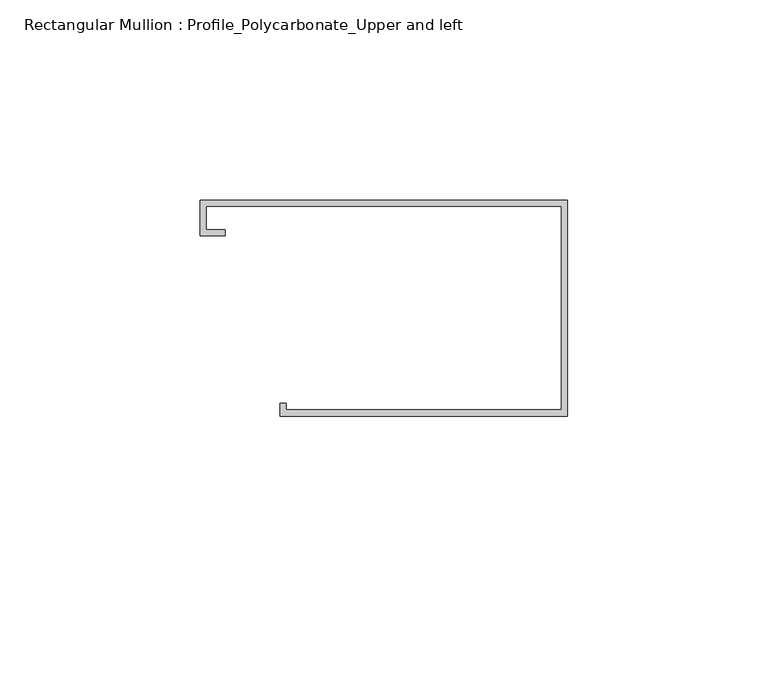
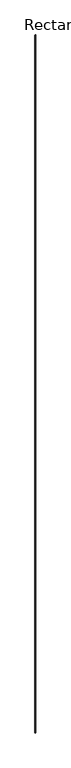
"""IFC4 building model written with IfcOpenShell, lengths in millimetres: member geometry, Rectangular Mullion : Profile_Polycarbonate_Upper and left."""

from ifc_helpers import new_model, si_unit, frame, origin, place, context, project, spatial, polyline, outline, extrude, source, transform, mapped, element, save


def rectangular_mullion_profile_polycarbonate_upper_and_left_873bee1a(model_context):
    return source(origin(), model_context, "Body", "SweptSolid", [
        extrude(outline(polyline([(0.0, 28.984575), (0.0, -25.015825), (-71.9836, -25.015825), (-71.9836, -21.840825), (-70.3961, -21.840825), (-70.3961, -23.428325), (-1.5875, -23.428325), (-1.5875, 27.397075), (-90.4113, 27.397075), (-90.4113, 21.580475), (-85.6488, 21.580475), (-85.6488, 19.992975), (-91.9988, 19.992975), (-91.9988, 28.984575), (0.0, 28.984575)])), frame((0.0, 0.0, -88779.5278), z_axis=(0.0, 0.0, 1.0), x_axis=(1.0, 0.0, 0.0)), (0.0, 0.0, 1.0), 88779.5278),
    ])


if __name__ == "__main__":
    model = new_model("IFC4")
    model_context = context("Model", 3, world=origin())
    ifc_project = project(units=[si_unit("LENGTHUNIT", "METRE", prefix="MILLI")], contexts=[model_context])
    site = spatial("IfcSite", under=ifc_project)
    building = spatial("IfcBuilding", under=site)
    placement = place(None, origin())
    rectangular_mullion_profile_polycarbonate_upper_and_left_shape = rectangular_mullion_profile_polycarbonate_upper_and_left_873bee1a(model_context)
    element("IfcMember", 1, ObjectType="Rectangular Mullion : Profile_Polycarbonate_Upper and left", at=placement, inside=building, context=model_context, shape_type="MappedRepresentation", body=[
        mapped(rectangular_mullion_profile_polycarbonate_upper_and_left_shape, transform((0.0, 0.0, 0.0), x_axis=(1.0, 0.0, 0.0), y_axis=(0.0, 1.0, 0.0), z_axis=(0.0, 0.0, 1.0))),
    ])
    save(model, "model.ifc")

# Revit data of these elements
# Type "Rectangular Mullion : Profile_Polycarbonate_Upper and left"
#   built-in parameter 1007322 = 0.177167 (stored number, unit not read)
#   built-in parameter 1007321 = 0.00520833 (stored number, unit not read)
#   built-in parameter 1007320 = 0 (stored number, unit not read)
